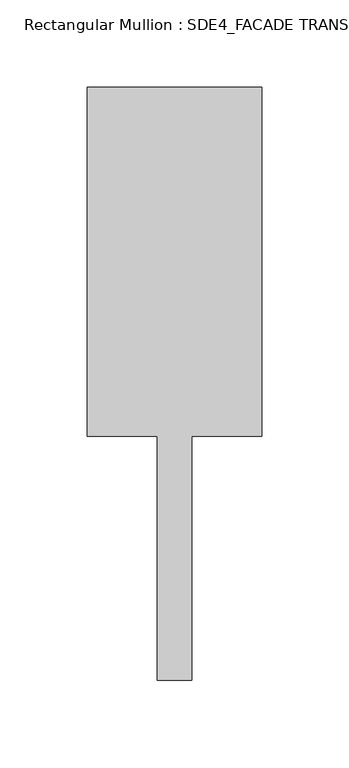
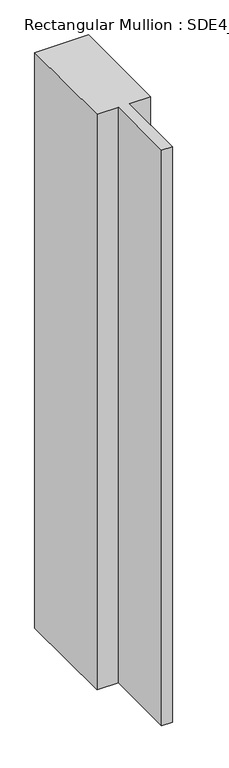
"""IFC4 building model written with IfcOpenShell, lengths in millimetres: member geometry, Rectangular Mullion : SDE4_FACADE TRANSOM TYPE 1."""

from ifc_helpers import new_model, si_unit, frame, origin, place, context, project, spatial, polyline, outline, extrude, source, transform, mapped, element, save


def rectangular_mullion_sde4_facade_transom_type_1_957d62d3(model_context):
    return source(origin(), model_context, "Body", "SweptSolid", [
        extrude(outline(polyline([(50.0, 132.5), (50.0, -67.5), (10.0, -67.5), (10.0, -207.5), (-10.0, -207.5), (-10.0, -67.5), (-50.0, -67.5), (-50.0, 132.5), (50.0, 132.5)])), frame((0.0, 0.0, -1131.5000001), z_axis=(0.0, 0.0, 1.0), x_axis=(1.0, 0.0, 0.0)), (0.0, 0.0, 1.0), 1131.5000001),
    ])


if __name__ == "__main__":
    model = new_model("IFC4")
    model_context = context("Model", 3, world=origin())
    ifc_project = project(units=[si_unit("LENGTHUNIT", "METRE", prefix="MILLI")], contexts=[model_context])
    site = spatial("IfcSite", under=ifc_project)
    building = spatial("IfcBuilding", under=site)
    placement = place(None, origin())
    rectangular_mullion_sde4_facade_transom_type_1_shape = rectangular_mullion_sde4_facade_transom_type_1_957d62d3(model_context)
    element("IfcMember", 1, ObjectType="Rectangular Mullion : SDE4_FACADE TRANSOM TYPE 1", at=placement, inside=building, context=model_context, shape_type="MappedRepresentation", body=[
        mapped(rectangular_mullion_sde4_facade_transom_type_1_shape, transform((0.0, 0.0, 0.0), x_axis=(1.0, 0.0, 0.0), y_axis=(0.0, 1.0, 0.0), z_axis=(0.0, 0.0, 1.0))),
    ])
    save(model, "model.ifc")

# Revit data of these elements
# Type "Rectangular Mullion : SDE4_FACADE TRANSOM TYPE 1"
#   built-in parameter 1007322 = 1.11549 (stored number, unit not read)
#   built-in parameter 1007321 = 0.164042 (stored number, unit not read)
#   built-in parameter 1007320 = 0.164042 (stored number, unit not read)
